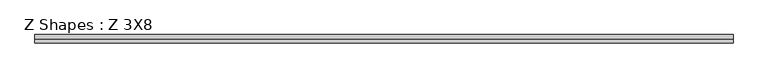
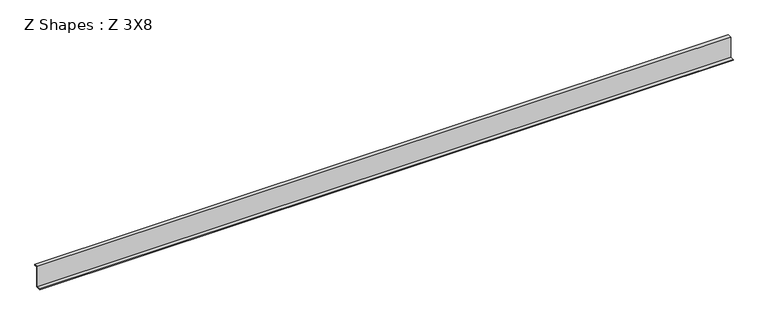
"""IFC4 building model written with IfcOpenShell, lengths in millimetres: beam geometry, Z Shapes : Z 3X8."""

from ifc_helpers import new_model, si_unit, frame, origin, place, context, project, spatial, polyline, outline, extrude, source, transform, mapped, element, save


def z_shapes_z_3x8_9c910b96(model_context):
    return source(origin(), model_context, "Body", "SweptSolid", [
        extrude(outline(polyline([(57.2805719, 92.452825), (27.1991352, 92.452825), (27.1991352, -98.809175), (-18.9194281, -98.809175), (-18.9194281, -92.459175), (19.1805719, -92.459175), (19.1805719, 102.104825), (57.2805719, 102.104825), (57.2805719, 92.452825)])), frame((-3168.6499994, 0.0, 0.0), z_axis=(1.0, 0.0, 0.0), x_axis=(0.0, 1.0, 0.0)), (0.0, 0.0, 1.0), 6337.2999994),
    ])


if __name__ == "__main__":
    model = new_model("IFC4")
    model_context = context("Model", 3, world=origin())
    ifc_project = project(units=[si_unit("LENGTHUNIT", "METRE", prefix="MILLI")], contexts=[model_context])
    site = spatial("IfcSite", under=ifc_project)
    building = spatial("IfcBuilding", under=site)
    placement = place(None, origin())
    z_shapes_z_3x8_shape = z_shapes_z_3x8_9c910b96(model_context)
    element("IfcBeam", 1, ObjectType="Z Shapes : Z 3X8", at=placement, inside=building, context=model_context, shape_type="MappedRepresentation", body=[
        mapped(z_shapes_z_3x8_shape, transform((0.0, 0.0, 0.0), x_axis=(1.0, 0.0, 0.0), y_axis=(0.0, 1.0, 0.0), z_axis=(0.0, 0.0, 1.0))),
    ])
    save(model, "model.ifc")

# Revit data of these elements
# Type "Z Shapes : Z 3X8"
#   Section Name Key = "W12x26"
#   Assembly Code = "B10"
#   Width = 76.2 mm
#   Web Thickness = 5.842 mm
#   Web Fillet = 7.62 mm
#   Warping Constant = 163001.3 cm⁶
#   Torsional Moment of Inertia = 12.4869 cm⁴
#   Section Area = 7.65 in²
#   Plastic Modulus weak axis = 0.00472801 (stored number, unit not read)
#   Plastic Modulus strong axis = 0.0215278 (stored number, unit not read)
#   Perimeter = 15.0571 m²/m
#   Nominal Weight = 379.441 N/m
#   Moment of Inertia weak axis = 720.08 cm⁴
#   Moment of Inertia strong axis = 8491.12 cm⁴
#   Height = 184.912 mm
#   Flange Thickness = 9.652 mm
#   Elastic Modulus weak axis = 0.00309028 (stored number, unit not read)
#   Elastic Modulus strong axis = 0.0193287 (stored number, unit not read)
#   Centroid Vertical = 92.456 mm
#   Centroid Horizontal = 38.1 mm
#   Length [instance default] = 5' - 0"
#   Structural Material [instance default] = Steel ASTM A992
#   Principal Axes Angle = 0
# Element 1 (IfcBeam, "Z Shapes : Z 3X8")
#   Structural Material = accent 2
#   Materials on its faces: "accent 2"
# Materials
#   "Steel ASTM A992": class "Metal", colour RGB 189 187 185, transparency 0, Description = "Structural steel 50ksi", Cost = 0
#   "accent 2": class "Wood", colour RGB 80 80 80, transparency 0, Description = "Wood framing, thermal airspace", Cost = 0
